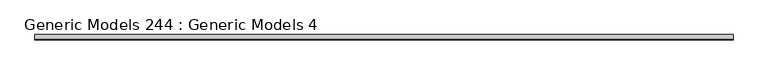
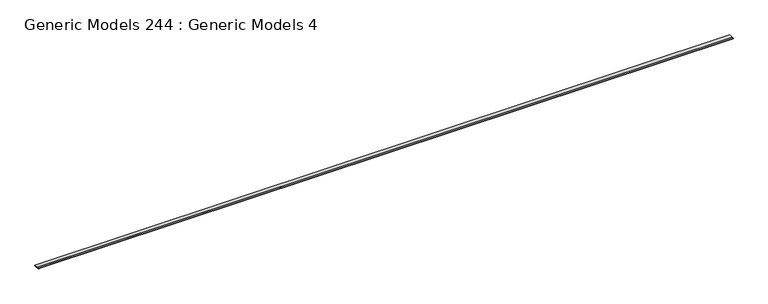
"""IFC4 building model written with IfcOpenShell, lengths in millimetres: proxy geometry, Generic Models 244 : Generic Models 4."""

from ifc_helpers import new_model, si_unit, origin, place, context, project, spatial, faceted_brep, source, transform, mapped, element, save


def generic_models_244_generic_models_4_af83e0b6(model_context):
    return source(origin(), model_context, "Body", "Brep", [
        faceted_brep([(8277.1941326, 11954.0420397, 126343.791), (8277.1941326, 11954.0420397, 126355.221), (8277.1941326, 11954.0420397, 126364.746), (8277.1941326, 11842.0673118, 126364.746), (8277.1941326, 11842.0673118, 126363.476), (8277.1941326, 11805.2373118, 126363.476), (8277.1941326, 11805.2373118, 126343.791), (8277.1941326, 11807.4471118, 126343.791), (8277.1941326, 11807.4471118, 126345.5234564), (8277.1941326, 11808.7171118, 126345.5234564), (8277.1941326, 11808.7171118, 126342.521), (8277.1941326, 11931.5988558, 126342.521), (8277.1941326, 11931.5988558, 126343.791), (-10366.4058674, 11954.0420397, 126364.746), (-10366.4058674, 11954.0420397, 126355.221), (-10366.4058674, 11954.0420397, 126343.791), (-10366.4058674, 11931.5988558, 126343.791), (-10366.4058674, 11931.5988558, 126342.521), (-10366.4058674, 11808.7171118, 126342.521), (-10366.4058674, 11808.7171118, 126345.5234564), (-10366.4058674, 11807.4471118, 126345.5234564), (-10366.4058674, 11807.4471118, 126343.791), (-10366.4058674, 11805.2373118, 126343.791), (-10366.4058674, 11805.2373118, 126363.476), (-10366.4058674, 11842.0673118, 126363.476), (-10366.4058674, 11842.0673118, 126364.746)], [[[0, 1, 2, 3, 4, 5, 6, 7, 8, 9, 10, 11, 12]], [[13, 14, 15, 16, 17, 18, 19, 20, 21, 22, 23, 24, 25]], [[2, 13, 25, 3]], [[17, 11, 10, 18]], [[13, 2, 1, 0, 15, 14]], [[16, 12, 11, 17]], [[12, 16, 15, 0]], [[24, 4, 3, 25]], [[4, 24, 23, 5]], [[5, 23, 22, 6]], [[6, 22, 21, 7]], [[8, 20, 19, 9]], [[9, 19, 18, 10]], [[20, 8, 7, 21]]]),
    ])


if __name__ == "__main__":
    model = new_model("IFC4")
    model_context = context("Model", 3, world=origin())
    ifc_project = project(units=[si_unit("LENGTHUNIT", "METRE", prefix="MILLI")], contexts=[model_context])
    site = spatial("IfcSite", under=ifc_project)
    building = spatial("IfcBuilding", under=site)
    placement = place(None, origin())
    generic_models_244_generic_models_4_shape = generic_models_244_generic_models_4_af83e0b6(model_context)
    element("IfcBuildingElementProxy", 1, Name="Generic Models 244 : Generic Models 4", ObjectType="Generic Models 244 : Generic Models 4", at=placement, inside=building, context=model_context, shape_type="MappedRepresentation", body=[
        mapped(generic_models_244_generic_models_4_shape, transform((0.0, 0.0, 0.0), x_axis=(1.0, 0.0, 0.0), y_axis=(0.0, 1.0, 0.0), z_axis=(0.0, 0.0, 1.0))),
    ])
    save(model, "model.ifc")

# Revit data of these elements
# Element 1 (IfcBuildingElementProxy, "Generic Models 244 : Generic Models 4")
#   Materials on its faces: "_7/8\" SMOOTH TROWEL EXTERIOR STUCCO (COLOR PER OWNER)"
# Materials
#   "_7/8\" SMOOTH TROWEL EXTERIOR STUCCO (COLOR PER OWNER)": class "Generic", colour RGB 233 233 233, transparency 0, Cost = 0
